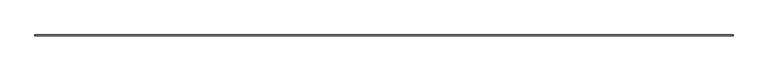
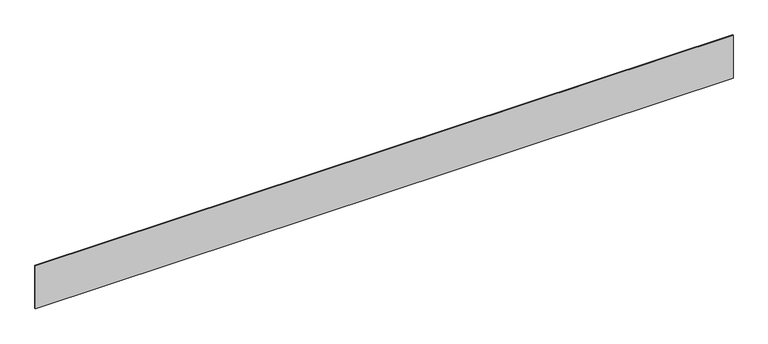
"""IFC4 building model written with IfcOpenShell, lengths in millimetres: proxy geometry, Inner panel:Inner panel:1:Inner panel:1 : Inner panel:Inner panel:300324:300043:Inner panel:1:Inner panel:1 : Inner panel:Inner panel:300324:300043 : Inner panel:Inner panel:1:Inner panel:1 : Inner panel:Inner panel:300324:300043:40 : Inner panel:Inner panel:1:Inner panel:1 : Inner panel:Inner panel:300324:300043:Inner panel:1:Inner panel:1 : Inner panel:Inner panel:300324:300043 : Inner panel:Inner panel:1:Inner panel:1 : Inner panel:Inner panel:300324:300043:300031."""

import ifcopenshell
import ifcopenshell.guid

model = None  # the IFC model being written
_history = None  # IfcOwnerHistory: only IFC2X3 demands one
_inside = {}  # id of a spatial element -> (the spatial element, [elements in it])
_under = {}  # id of a project, library or spatial element -> (it, [spatial elements below it])
_declared = {}  # id of a project -> (the project, [libraries it declares])
_typed = {}  # id of a type object -> (the type object, [elements of that type])
_made_of = {}  # id of a material, layer set ... -> (it, [elements and type objects made of it])


def new_model(schema):
    """Start an empty IFC model of exactly this schema.

    Asked for "IFC4X3", IfcOpenShell would pick the latest addendum, in which some entities
    have other attributes; the version numbers below select the first issue.
    IFC2X3 requires an IfcOwnerHistory on every rooted entity: one is made here for all.
    """
    global model, _history
    if schema == "IFC4X3":
        model = ifcopenshell.file(schema_version=(4, 3, 0, 0))
    else:
        model = ifcopenshell.file(schema=schema)
    _inside.clear()
    _under.clear()
    _declared.clear()
    _typed.clear()
    _made_of.clear()
    _history = None
    if model.schema == "IFC2X3":
        org = make("IfcOrganization", Name="unknown")
        user = make(
            "IfcPersonAndOrganization",
            ThePerson=make("IfcPerson", FamilyName="unknown"),
            TheOrganization=org,
        )
        app = make(
            "IfcApplication",
            ApplicationDeveloper=org,
            Version="unknown",
            ApplicationFullName="unknown",
            ApplicationIdentifier="unknown",
        )
        _history = make(
            "IfcOwnerHistory",
            OwningUser=user,
            OwningApplication=app,
            ChangeAction="ADDED",
            CreationDate=0,
        )
    return model


def make(cls, **values):
    """One entity of the class cls with the attributes given. An attribute that is None is left unset."""
    return model.create_entity(
        cls, **{name: value for name, value in values.items() if value is not None}
    )


def rooted(cls, **values):
    """An entity with a GlobalId (a new one), such as an element, a storey or a relation."""
    return make(cls, GlobalId=ifcopenshell.guid.new(), OwnerHistory=_history, **values)


def si_unit(unit_type, name, prefix=None):
    """IfcSIUnit, for example si_unit("LENGTHUNIT", "METRE", prefix="MILLI")."""
    return make("IfcSIUnit", UnitType=unit_type, Prefix=prefix, Name=name)


def assignment(units):
    """IfcUnitAssignment: the units of a project."""
    return None if units is None else make("IfcUnitAssignment", Units=units)


def point(xyz):
    """IfcCartesianPoint."""
    return None if xyz is None else make("IfcCartesianPoint", Coordinates=xyz)


def direction(xyz):
    """IfcDirection."""
    return None if xyz is None else make("IfcDirection", DirectionRatios=xyz)


def frame(location, z_axis=None, x_axis=None):
    """IfcAxis2Placement3D, a coordinate frame: its origin and axes. An axis left out is left unset."""
    return make(
        "IfcAxis2Placement3D",
        Location=point(location),
        Axis=direction(z_axis),
        RefDirection=direction(x_axis),
    )


def origin():
    """The frame at (0, 0, 0) with its axes left unset."""
    return frame((0.0, 0.0, 0.0))


def place(relative_to, where):
    """IfcLocalPlacement: puts the frame where relative to a parent placement (None: the world)."""
    return make(
        "IfcLocalPlacement", PlacementRelTo=relative_to, RelativePlacement=where
    )


def context(
    kind, dimensions, precision=None, world=None, true_north=None, identifier=None
):
    """IfcGeometricRepresentationContext, for example the 3D "Model" context."""
    return make(
        "IfcGeometricRepresentationContext",
        ContextIdentifier=identifier,
        ContextType=kind,
        CoordinateSpaceDimension=dimensions,
        Precision=precision,
        WorldCoordinateSystem=world,
        TrueNorth=true_north,
    )


def project(units=None, contexts=None):
    """IfcProject with its units and contexts."""
    return rooted(
        "IfcProject",
        Name="project",
        RepresentationContexts=contexts,
        UnitsInContext=assignment(units),
    )


def spatial(cls, under=None, at=None, **own):
    """A site, building, storey or space (cls), placed at a placement, below another one or the project."""
    s = rooted(cls, ObjectPlacement=at, **own)
    if under is not None:
        _under.setdefault(under.id(), (under, []))[1].append(s)
    return s


def polyline(points):
    """IfcPolyline through the points."""
    return make("IfcPolyline", Points=[point(p) for p in points])


def outline(outer, holes=None, kind="AREA"):
    """IfcArbitraryClosedProfileDef: a profile drawn as a closed curve; with holes, ...WithVoids."""
    if holes is None:
        return make("IfcArbitraryClosedProfileDef", ProfileType=kind, OuterCurve=outer)
    return make(
        "IfcArbitraryProfileDefWithVoids",
        ProfileType=kind,
        OuterCurve=outer,
        InnerCurves=holes,
    )


def extrude(swept, where, along, depth):
    """IfcExtrudedAreaSolid: the profile swept, set in the frame where, extruded along a direction by depth."""
    return make(
        "IfcExtrudedAreaSolid",
        SweptArea=swept,
        Position=where,
        ExtrudedDirection=direction(along),
        Depth=depth,
    )


def shape(context_of_items, identifier, shape_type, items):
    """IfcShapeRepresentation: the items that make up one representation, for example the "Body"."""
    return make(
        "IfcShapeRepresentation",
        ContextOfItems=context_of_items,
        RepresentationIdentifier=identifier,
        RepresentationType=shape_type,
        Items=items,
    )


def source(mapping_origin, context_of_items, identifier, shape_type, items):
    """IfcRepresentationMap: a shape defined once, which mapped items show again and again."""
    return make(
        "IfcRepresentationMap",
        MappingOrigin=mapping_origin,
        MappedRepresentation=shape(context_of_items, identifier, shape_type, items),
    )


def transform(
    local_origin,
    x_axis=None,
    y_axis=None,
    z_axis=None,
    scale=None,
    scale2=None,
    scale3=None,
    uniform=True,
):
    """IfcCartesianTransformationOperator3D, or its non-uniform kind. x_axis, y_axis, z_axis: its Axis1, 2, 3."""
    if uniform:
        return make(
            "IfcCartesianTransformationOperator3D",
            Axis1=direction(x_axis),
            Axis2=direction(y_axis),
            LocalOrigin=point(local_origin),
            Scale=scale,
            Axis3=direction(z_axis),
        )
    return make(
        "IfcCartesianTransformationOperator3DnonUniform",
        Axis1=direction(x_axis),
        Axis2=direction(y_axis),
        LocalOrigin=point(local_origin),
        Scale=scale,
        Axis3=direction(z_axis),
        Scale2=scale2,
        Scale3=scale3,
    )


def mapped(mapping_source, mapping_target):
    """IfcMappedItem: shows the shape of a source again, moved by a transform."""
    return make(
        "IfcMappedItem", MappingSource=mapping_source, MappingTarget=mapping_target
    )


def made_of(thing, what):
    """Note that an element or type object is made of a material, layer set ...; save() writes the relation."""
    if what is not None:
        _made_of.setdefault(what.id(), (what, []))[1].append(thing)
    return thing


def element(
    cls,
    number,
    at=None,
    inside=None,
    cuts=None,
    type_object=None,
    material=None,
    context=None,
    identifier="Body",
    shape_type=None,
    held_by="IfcProductDefinitionShape",
    body=None,
    shapes=None,
    **own,
):
    """One element of the class cls, such as IfcWall. Its Tag is "e" and its number.

    at: its placement. inside: the storey or other place that contains it. cuts: it is an
    opening in that element (IfcRelVoidsElement). A single representation is given by context,
    identifier, shape_type and body (its items); several are given by shapes. held_by: the class
    of the entity that holds the representations. save() writes the other relations.
    """
    e = rooted(cls, Tag="e%d" % number, ObjectPlacement=at, **own)
    if body is not None:
        shapes = [shape(context, identifier, shape_type, body)]
    if shapes is not None:
        e.Representation = make(held_by, Representations=shapes)
    if inside is not None:
        _inside.setdefault(inside.id(), (inside, []))[1].append(e)
    if cuts is not None:
        rooted(
            "IfcRelVoidsElement", RelatingBuildingElement=cuts, RelatedOpeningElement=e
        )
    if type_object is not None:
        _typed.setdefault(type_object.id(), (type_object, []))[1].append(e)
    return made_of(e, material)


def aggregate(whole, parts):
    """IfcRelAggregates: a whole, such as a stair, and the parts it consists of."""
    return rooted("IfcRelAggregates", RelatingObject=whole, RelatedObjects=parts)


def save(model, path):
    """Write the relations noted so far, then the file.

    IfcRelAggregates (storeys below a building ...), IfcRelContainedInSpatialStructure (elements
    in a storey), IfcRelDefinesByType, IfcRelAssociatesMaterial and IfcRelDeclares: one each for
    every whole, place, type object, material and project.
    """
    for whole, parts in _under.values():
        aggregate(whole, parts)
    for where, things in _inside.values():
        rooted(
            "IfcRelContainedInSpatialStructure",
            RelatedElements=things,
            RelatingStructure=where,
        )
    for kind, things in _typed.values():
        rooted("IfcRelDefinesByType", RelatedObjects=things, RelatingType=kind)
    for what, things in _made_of.values():
        rooted("IfcRelAssociatesMaterial", RelatedObjects=things, RelatingMaterial=what)
    for by, libraries in _declared.values():
        rooted("IfcRelDeclares", RelatingContext=by, RelatedDefinitions=libraries)
    model.write(path)


def generic_models_62b4d815(model_context):
    return source(origin(), model_context, "Body", "SweptSolid", [
        extrude(outline(polyline([(560352.9617239, -578778.4413841), (579104.5117239, -578778.4413841), (579104.5117239, -578797.4913841), (560352.9617239, -578797.4913841), (560352.9617239, -578778.4413841)])), frame((0.0, 0.0, 4946.65), z_axis=(0.0, 0.0, 1.0), x_axis=(1.0, 0.0, 0.0)), (0.0, 0.0, 1.0), 1219.2),
    ])


if __name__ == "__main__":
    model = new_model("IFC4")
    model_context = context("Model", 3, world=origin())
    ifc_project = project(units=[si_unit("LENGTHUNIT", "METRE", prefix="MILLI")], contexts=[model_context])
    site = spatial("IfcSite", under=ifc_project)
    building = spatial("IfcBuilding", under=site)
    placement = place(None, origin())
    generic_models_shape = generic_models_62b4d815(model_context)
    element("IfcBuildingElementProxy", 1, Name="Inner panel:Inner panel:1:Inner panel:1 : Inner panel:Inner panel:300324:300043:Inner panel:1:Inner panel:1 : Inner panel:Inner panel:300324:300043 : Inner panel:Inner panel:1:Inner panel:1 : Inner panel:Inner panel:300324:300043:40 : Inner panel:Inner panel:1:Inner panel:1 : Inner panel:Inner panel:300324:300043:Inner panel:1:Inner panel:1 : Inner panel:Inner panel:300324:300043 : Inner panel:Inner panel:1:Inner panel:1 : Inner panel:Inner panel:300324:300043:300031", ObjectType="Inner panel:Inner panel:1:Inner panel:1 : Inner panel:Inner panel:300324:300043:Inner panel:1:Inner panel:1 : Inner panel:Inner panel:300324:300043 : Inner panel:Inner panel:1:Inner panel:1 : Inner panel:Inner panel:300324:300043:40 : Inner panel:Inner panel:1:Inner panel:1 : Inner panel:Inner panel:300324:300043:Inner panel:1:Inner panel:1 : Inner panel:Inner panel:300324:300043 : Inner panel:Inner panel:1:Inner panel:1 : Inner panel:Inner panel:300324:300043:300031", at=placement, inside=building, context=model_context, shape_type="MappedRepresentation", body=[
        mapped(generic_models_shape, transform((0.0, 0.0, 0.0), x_axis=(1.0, 0.0, 0.0), y_axis=(0.0, 1.0, 0.0), z_axis=(0.0, 0.0, 1.0))),
    ])
    save(model, "model.ifc")

# Revit data of these elements
# Type "Inner panel:Inner panel:1:Inner panel:1 : Inner panel:Inner panel:300324:300043:Inner panel:1:Inner panel:1 : Inner panel:Inner panel:300324:300043 : Inner panel:Inner panel:1:Inner panel:1 : Inner panel:Inner panel:300324:300043:40 : Inner panel:Inner panel:1:Inner panel:1 : Inner panel:Inner panel:300324:300043:Inner panel:1:Inner panel:1 : Inner panel:Inner panel:300324:300043 : Inner panel:Inner panel:1:Inner panel:1 : Inner panel:Inner panel:300324:300043:300031"
#   NameOverride = "Inner panel:Inner panel:1:Inner panel:1 : Inner panel:Inner panel:300324:300043:Inner panel:1:Inner panel:1 : Inner panel:Inner panel:300324:300043 : Inner panel:Inner panel:1:Inner panel:1 : Inner panel:Inner panel:300324:300043:300031"
#   ObjectTypeOverride = "Inner panel:1:Inner panel:1 : Inner panel:Inner panel:300324:300043 : Inner panel:Inner panel:1:Inner panel:1 : Inner panel:Inner panel:300324:300043"
#   Reference = "Inner panel"
#   Tag = "300031"
# Element 1 (IfcBuildingElementProxy, "Inner panel:Inner panel:1:Inner panel:1 : Inner panel:Inner panel:300324:300043:Inner panel:1:Inner panel:1 : Inner panel:Inner panel:300324:300043 : Inner panel:Inner panel:1:Inner panel:1 : Inner panel:Inner panel:300324:300043:40 : Inner panel:Inner panel:1:Inner panel:1 : Inner panel:Inner panel:300324:300043:Inner panel:1:Inner panel:1 : Inner panel:Inner panel:300324:300043 : Inner panel:Inner panel:1:Inner panel:1 : Inner panel:Inner panel:300324:300043:300031")
#   Materials on its faces: "3/4\" EXTERIOR GRADE FIRE RETARDANT PLYWOOD (FINISH: GRADE B)"
# Materials
#   "3/4\" EXTERIOR GRADE FIRE RETARDANT PLYWOOD (FINISH: GRADE B)": class "Wood", colour RGB 149 120 74, transparency 0, Description = "Plywood, sheathing grade", Cost = 0
